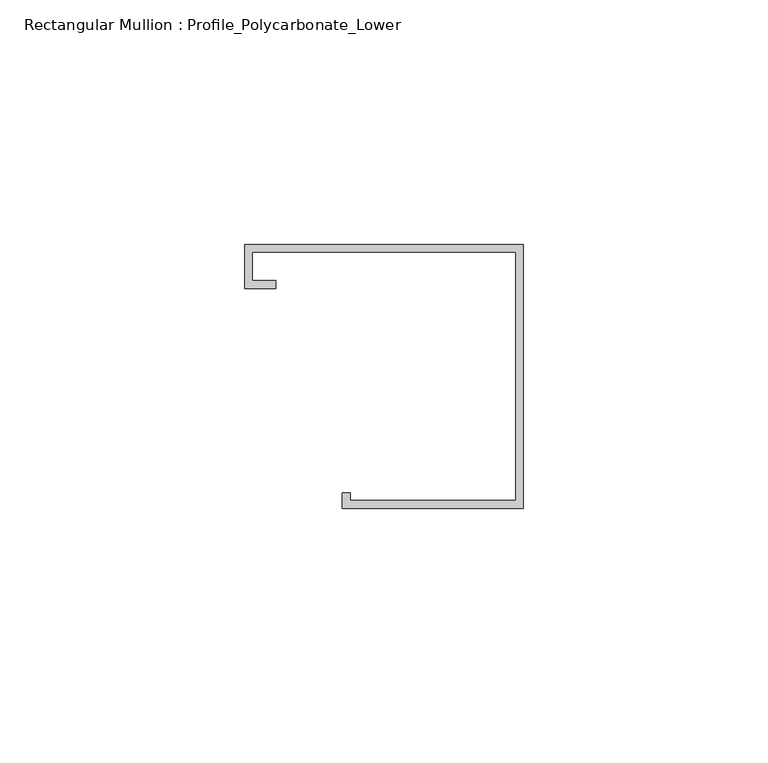
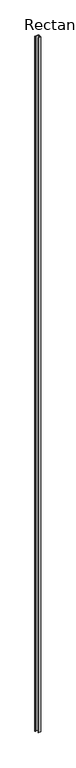
"""IFC4 building model written with IfcOpenShell, lengths in millimetres: member geometry, Rectangular Mullion : Profile_Polycarbonate_Lower."""

from ifc_helpers import new_model, si_unit, frame, origin, place, context, project, spatial, polyline, outline, extrude, source, transform, mapped, element, save


def rectangular_mullion_profile_polycarbonate_lower_d4e25c84(model_context):
    return source(origin(), model_context, "Body", "SweptSolid", [
        extrude(outline(polyline([(0.0, 28.984575), (0.0, -25.015825), (-36.9824, -25.015825), (-36.9824, -21.840825), (-35.3949, -21.840825), (-35.3949, -23.428325), (-1.5875, -23.428325), (-1.5875, 27.397075), (-55.4101, 27.397075), (-55.4101, 21.580475), (-50.6476, 21.580475), (-50.6476, 19.992975), (-56.9976, 19.992975), (-56.9976, 28.984575), (0.0, 28.984575)])), frame((0.0, 0.0, -11382.5274), z_axis=(0.0, 0.0, 1.0), x_axis=(1.0, 0.0, 0.0)), (0.0, 0.0, 1.0), 11382.5274),
    ])


if __name__ == "__main__":
    model = new_model("IFC4")
    model_context = context("Model", 3, world=origin())
    ifc_project = project(units=[si_unit("LENGTHUNIT", "METRE", prefix="MILLI")], contexts=[model_context])
    site = spatial("IfcSite", under=ifc_project)
    building = spatial("IfcBuilding", under=site)
    placement = place(None, origin())
    rectangular_mullion_profile_polycarbonate_lower_shape = rectangular_mullion_profile_polycarbonate_lower_d4e25c84(model_context)
    element("IfcMember", 1, ObjectType="Rectangular Mullion : Profile_Polycarbonate_Lower", at=placement, inside=building, context=model_context, shape_type="MappedRepresentation", body=[
        mapped(rectangular_mullion_profile_polycarbonate_lower_shape, transform((0.0, 0.0, 0.0), x_axis=(1.0, 0.0, 0.0), y_axis=(0.0, 1.0, 0.0), z_axis=(0.0, 0.0, 1.0))),
    ])
    save(model, "model.ifc")

# Revit data of these elements
# Type "Rectangular Mullion : Profile_Polycarbonate_Lower"
#   built-in parameter 1007322 = 0.177167 (stored number, unit not read)
#   built-in parameter 1007321 = 0 (stored number, unit not read)
#   built-in parameter 1007320 = 0.00520833 (stored number, unit not read)
